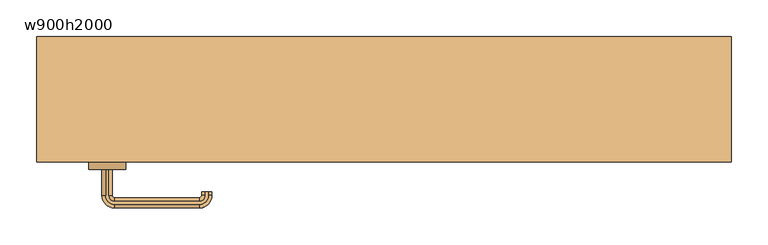
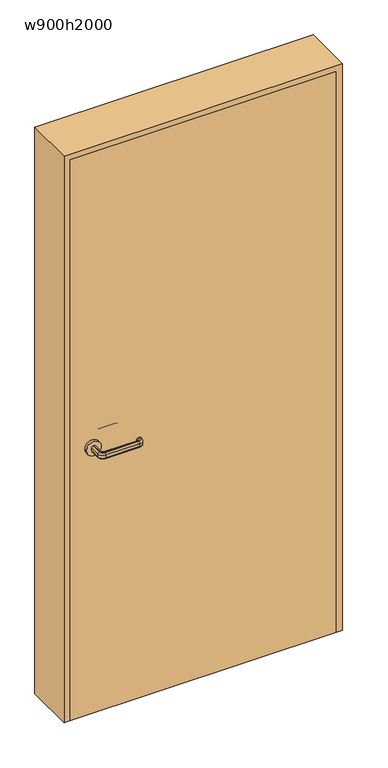
"""IFC4 building model written with IfcOpenShell, lengths in millimetres: door geometry, 片開き : w900h2000."""

import ifcopenshell
import ifcopenshell.guid

model = None  # the IFC model being written
_history = None  # IfcOwnerHistory: only IFC2X3 demands one
_inside = {}  # id of a spatial element -> (the spatial element, [elements in it])
_under = {}  # id of a project, library or spatial element -> (it, [spatial elements below it])
_declared = {}  # id of a project -> (the project, [libraries it declares])
_typed = {}  # id of a type object -> (the type object, [elements of that type])
_made_of = {}  # id of a material, layer set ... -> (it, [elements and type objects made of it])


def new_model(schema):
    """Start an empty IFC model of exactly this schema.

    Asked for "IFC4X3", IfcOpenShell would pick the latest addendum, in which some entities
    have other attributes; the version numbers below select the first issue.
    IFC2X3 requires an IfcOwnerHistory on every rooted entity: one is made here for all.
    """
    global model, _history
    if schema == "IFC4X3":
        model = ifcopenshell.file(schema_version=(4, 3, 0, 0))
    else:
        model = ifcopenshell.file(schema=schema)
    _inside.clear()
    _under.clear()
    _declared.clear()
    _typed.clear()
    _made_of.clear()
    _history = None
    if model.schema == "IFC2X3":
        org = make("IfcOrganization", Name="unknown")
        user = make(
            "IfcPersonAndOrganization",
            ThePerson=make("IfcPerson", FamilyName="unknown"),
            TheOrganization=org,
        )
        app = make(
            "IfcApplication",
            ApplicationDeveloper=org,
            Version="unknown",
            ApplicationFullName="unknown",
            ApplicationIdentifier="unknown",
        )
        _history = make(
            "IfcOwnerHistory",
            OwningUser=user,
            OwningApplication=app,
            ChangeAction="ADDED",
            CreationDate=0,
        )
    return model


def make(cls, **values):
    """One entity of the class cls with the attributes given. An attribute that is None is left unset."""
    return model.create_entity(
        cls, **{name: value for name, value in values.items() if value is not None}
    )


def rooted(cls, **values):
    """An entity with a GlobalId (a new one), such as an element, a storey or a relation."""
    return make(cls, GlobalId=ifcopenshell.guid.new(), OwnerHistory=_history, **values)


def si_unit(unit_type, name, prefix=None):
    """IfcSIUnit, for example si_unit("LENGTHUNIT", "METRE", prefix="MILLI")."""
    return make("IfcSIUnit", UnitType=unit_type, Prefix=prefix, Name=name)


def assignment(units):
    """IfcUnitAssignment: the units of a project."""
    return None if units is None else make("IfcUnitAssignment", Units=units)


def point(xyz):
    """IfcCartesianPoint."""
    return None if xyz is None else make("IfcCartesianPoint", Coordinates=xyz)


def direction(xyz):
    """IfcDirection."""
    return None if xyz is None else make("IfcDirection", DirectionRatios=xyz)


def frame(location, z_axis=None, x_axis=None):
    """IfcAxis2Placement3D, a coordinate frame: its origin and axes. An axis left out is left unset."""
    return make(
        "IfcAxis2Placement3D",
        Location=point(location),
        Axis=direction(z_axis),
        RefDirection=direction(x_axis),
    )


def frame_2d(location, x_axis=None):
    """IfcAxis2Placement2D, a coordinate frame in the plane: its origin and x axis."""
    return make(
        "IfcAxis2Placement2D", Location=point(location), RefDirection=direction(x_axis)
    )


def origin():
    """The frame at (0, 0, 0) with its axes left unset."""
    return frame((0.0, 0.0, 0.0))


def origin_with_axes():
    """The frame at (0, 0, 0) with the z axis (0, 0, 1) and the x axis (1, 0, 0) written out."""
    return frame((0.0, 0.0, 0.0), z_axis=(0.0, 0.0, 1.0), x_axis=(1.0, 0.0, 0.0))


def place(relative_to, where):
    """IfcLocalPlacement: puts the frame where relative to a parent placement (None: the world)."""
    return make(
        "IfcLocalPlacement", PlacementRelTo=relative_to, RelativePlacement=where
    )


def context(
    kind, dimensions, precision=None, world=None, true_north=None, identifier=None
):
    """IfcGeometricRepresentationContext, for example the 3D "Model" context."""
    return make(
        "IfcGeometricRepresentationContext",
        ContextIdentifier=identifier,
        ContextType=kind,
        CoordinateSpaceDimension=dimensions,
        Precision=precision,
        WorldCoordinateSystem=world,
        TrueNorth=true_north,
    )


def project(units=None, contexts=None):
    """IfcProject with its units and contexts."""
    return rooted(
        "IfcProject",
        Name="project",
        RepresentationContexts=contexts,
        UnitsInContext=assignment(units),
    )


def spatial(cls, under=None, at=None, **own):
    """A site, building, storey or space (cls), placed at a placement, below another one or the project."""
    s = rooted(cls, ObjectPlacement=at, **own)
    if under is not None:
        _under.setdefault(under.id(), (under, []))[1].append(s)
    return s


def polyline(points):
    """IfcPolyline through the points."""
    return make("IfcPolyline", Points=[point(p) for p in points])


def circle_curve(where, radius):
    """IfcCircle in the frame where."""
    return make("IfcCircle", Position=where, Radius=radius)


def ellipse_curve(where, semi_axis1, semi_axis2):
    """IfcEllipse in the frame where."""
    return make(
        "IfcEllipse", Position=where, SemiAxis1=semi_axis1, SemiAxis2=semi_axis2
    )


def trimmed(basis, trim1, trim2, sense, master):
    """IfcTrimmedCurve: the piece of a basis curve between two trims."""
    return make(
        "IfcTrimmedCurve",
        BasisCurve=basis,
        Trim1=trim1,
        Trim2=trim2,
        SenseAgreement=sense,
        MasterRepresentation=master,
    )


def segment(curve, same_sense, transition):
    """IfcCompositeCurveSegment."""
    return make(
        "IfcCompositeCurveSegment",
        Transition=transition,
        SameSense=same_sense,
        ParentCurve=curve,
    )


def composite_curve(segments, self_intersect=None):
    """IfcCompositeCurve: segments joined end to end."""
    return make("IfcCompositeCurve", Segments=segments, SelfIntersect=self_intersect)


def outline(outer, holes=None, kind="AREA"):
    """IfcArbitraryClosedProfileDef: a profile drawn as a closed curve; with holes, ...WithVoids."""
    if holes is None:
        return make("IfcArbitraryClosedProfileDef", ProfileType=kind, OuterCurve=outer)
    return make(
        "IfcArbitraryProfileDefWithVoids",
        ProfileType=kind,
        OuterCurve=outer,
        InnerCurves=holes,
    )


def extrude(swept, where, along, depth):
    """IfcExtrudedAreaSolid: the profile swept, set in the frame where, extruded along a direction by depth."""
    return make(
        "IfcExtrudedAreaSolid",
        SweptArea=swept,
        Position=where,
        ExtrudedDirection=direction(along),
        Depth=depth,
    )


def shape(context_of_items, identifier, shape_type, items):
    """IfcShapeRepresentation: the items that make up one representation, for example the "Body"."""
    return make(
        "IfcShapeRepresentation",
        ContextOfItems=context_of_items,
        RepresentationIdentifier=identifier,
        RepresentationType=shape_type,
        Items=items,
    )


def source(mapping_origin, context_of_items, identifier, shape_type, items):
    """IfcRepresentationMap: a shape defined once, which mapped items show again and again."""
    return make(
        "IfcRepresentationMap",
        MappingOrigin=mapping_origin,
        MappedRepresentation=shape(context_of_items, identifier, shape_type, items),
    )


def transform(
    local_origin,
    x_axis=None,
    y_axis=None,
    z_axis=None,
    scale=None,
    scale2=None,
    scale3=None,
    uniform=True,
):
    """IfcCartesianTransformationOperator3D, or its non-uniform kind. x_axis, y_axis, z_axis: its Axis1, 2, 3."""
    if uniform:
        return make(
            "IfcCartesianTransformationOperator3D",
            Axis1=direction(x_axis),
            Axis2=direction(y_axis),
            LocalOrigin=point(local_origin),
            Scale=scale,
            Axis3=direction(z_axis),
        )
    return make(
        "IfcCartesianTransformationOperator3DnonUniform",
        Axis1=direction(x_axis),
        Axis2=direction(y_axis),
        LocalOrigin=point(local_origin),
        Scale=scale,
        Axis3=direction(z_axis),
        Scale2=scale2,
        Scale3=scale3,
    )


def mapped(mapping_source, mapping_target):
    """IfcMappedItem: shows the shape of a source again, moved by a transform."""
    return make(
        "IfcMappedItem", MappingSource=mapping_source, MappingTarget=mapping_target
    )


def made_of(thing, what):
    """Note that an element or type object is made of a material, layer set ...; save() writes the relation."""
    if what is not None:
        _made_of.setdefault(what.id(), (what, []))[1].append(thing)
    return thing


def element(
    cls,
    number,
    at=None,
    inside=None,
    cuts=None,
    type_object=None,
    material=None,
    context=None,
    identifier="Body",
    shape_type=None,
    held_by="IfcProductDefinitionShape",
    body=None,
    shapes=None,
    **own,
):
    """One element of the class cls, such as IfcWall. Its Tag is "e" and its number.

    at: its placement. inside: the storey or other place that contains it. cuts: it is an
    opening in that element (IfcRelVoidsElement). A single representation is given by context,
    identifier, shape_type and body (its items); several are given by shapes. held_by: the class
    of the entity that holds the representations. save() writes the other relations.
    """
    e = rooted(cls, Tag="e%d" % number, ObjectPlacement=at, **own)
    if body is not None:
        shapes = [shape(context, identifier, shape_type, body)]
    if shapes is not None:
        e.Representation = make(held_by, Representations=shapes)
    if inside is not None:
        _inside.setdefault(inside.id(), (inside, []))[1].append(e)
    if cuts is not None:
        rooted(
            "IfcRelVoidsElement", RelatingBuildingElement=cuts, RelatedOpeningElement=e
        )
    if type_object is not None:
        _typed.setdefault(type_object.id(), (type_object, []))[1].append(e)
    return made_of(e, material)


def aggregate(whole, parts):
    """IfcRelAggregates: a whole, such as a stair, and the parts it consists of."""
    return rooted("IfcRelAggregates", RelatingObject=whole, RelatedObjects=parts)


def save(model, path):
    """Write the relations noted so far, then the file.

    IfcRelAggregates (storeys below a building ...), IfcRelContainedInSpatialStructure (elements
    in a storey), IfcRelDefinesByType, IfcRelAssociatesMaterial and IfcRelDeclares: one each for
    every whole, place, type object, material and project.
    """
    for whole, parts in _under.values():
        aggregate(whole, parts)
    for where, things in _inside.values():
        rooted(
            "IfcRelContainedInSpatialStructure",
            RelatedElements=things,
            RelatingStructure=where,
        )
    for kind, things in _typed.values():
        rooted("IfcRelDefinesByType", RelatedObjects=things, RelatingType=kind)
    for what, things in _made_of.values():
        rooted("IfcRelAssociatesMaterial", RelatedObjects=things, RelatingMaterial=what)
    for by, libraries in _declared.values():
        rooted("IfcRelDeclares", RelatingContext=by, RelatedDefinitions=libraries)
    model.write(path)


def plane_surface(at):
    """IfcPlane: the flat surface through the origin of the frame at, square to its z axis."""
    return make("IfcPlane", Position=at)


def cylinder_surface(at, radius):
    """IfcCylindricalSurface: all points at the distance radius from the z axis of the frame at."""
    return make("IfcCylindricalSurface", Position=at, Radius=radius)


def revolved_surface(curve, axis_point, axis_direction):
    """IfcSurfaceOfRevolution: the curve turned about the line through axis_point along axis_direction."""
    return make(
        "IfcSurfaceOfRevolution",
        SweptCurve=make("IfcArbitraryOpenProfileDef", ProfileType="CURVE", Curve=curve),
        AxisPosition=make("IfcAxis1Placement", Location=point(axis_point), Axis=direction(axis_direction)),
    )


def advanced_brep(points, edges, surfaces, faces):
    """IfcAdvancedBrep: a solid bounded by faces that lie on surfaces and meet in shared edges.

    An edge is (start, end): straight between two places in points (the first is 0);
    or (start, end, curve); or (start, end, curve, False) where it runs against its curve.
    A face is (place in surfaces, loops), or (place, loops, False) where it looks against
    its surface's normal. A loop lists edges by number (the first is 1), with a minus sign
    where the edge is run from its end to its start. The first loop is the outer one.
    """
    corners = [point(p) for p in points]
    vertices = [make("IfcVertexPoint", VertexGeometry=c) for c in corners]
    made = []
    for start, end, *more in edges:
        made.append(
            make(
                "IfcEdgeCurve",
                EdgeStart=vertices[start],
                EdgeEnd=vertices[end],
                EdgeGeometry=more[0] if more else make("IfcPolyline", Points=[corners[start], corners[end]]),
                SameSense=more[1] if len(more) > 1 else True,
            )
        )
    hull = []
    for where, loops, *sense in faces:
        bounds = []
        for j, loop in enumerate(loops):
            ring = [make("IfcOrientedEdge", EdgeElement=made[abs(k) - 1], Orientation=k > 0) for k in loop]
            bounds.append(
                make(
                    "IfcFaceOuterBound" if j == 0 else "IfcFaceBound",
                    Bound=make("IfcEdgeLoop", EdgeList=ring),
                    Orientation=True,
                )
            )
        hull.append(make("IfcAdvancedFace", Bounds=bounds, FaceSurface=surfaces[where], SameSense=sense[0] if sense else True))
    return make("IfcAdvancedBrep", Outer=make("IfcClosedShell", CfsFaces=hull))


def w900h2000_c063673d(model_context):
    return source(origin(), model_context, "Body", "SolidModel", [
        advanced_brep(
        [(-377.0, -95.0, 960.0), (-373.0, -95.0, 960.0), (-368.0, -95.0, 955.0), (-368.0, -95.0, 945.0477623), (-373.0, -95.0, 940.0477623), (-377.0, -95.0, 940.0477623), (-382.0, -95.0, 945.0477623), (-382.0, -95.0, 955.0), (-382.0, -130.0, 955.0), (-377.0, -130.0, 960.0), (-382.0, -130.0, 945.0477623), (-377.0, -130.0, 940.0477623), (-373.0, -130.0, 940.0477623), (-365.0, -138.0, 940.0477623), (-250.0, -138.0, 940.0477623), (-242.0, -130.0, 940.0477623), (-242.0, -125.0, 940.0477623), (-238.0, -125.0, 940.0477623), (-238.0, -130.0, 940.0477623), (-250.0, -142.0, 940.0477623), (-365.0, -142.0, 940.0477623), (-368.0, -130.0, 945.0477623), (-368.0, -130.0, 955.0), (-373.0, -130.0, 960.0), (-365.0, -142.0, 960.0), (-250.0, -142.0, 960.0), (-238.0, -130.0, 960.0), (-238.0, -125.0, 960.0), (-242.0, -125.0, 960.0), (-242.0, -130.0, 960.0), (-250.0, -138.0, 960.0), (-365.0, -138.0, 960.0), (-365.0, -147.0, 955.0), (-365.0, -147.0, 945.0477623), (-365.0, -133.0, 945.0477623), (-365.0, -133.0, 955.0), (-250.0, -147.0, 955.0), (-250.0, -147.0, 945.0477623), (-250.0, -133.0, 945.0477623), (-250.0, -133.0, 955.0), (-233.0, -130.0, 955.0), (-233.0, -130.0, 945.0477623), (-247.0, -130.0, 945.0477623), (-247.0, -130.0, 955.0), (-233.0, -125.0, 955.0), (-233.0, -125.0, 945.0477623), (-247.0, -125.0, 945.0477623), (-247.0, -125.0, 955.0)],
        [
            (0, 1),
            (1, 2, circle_curve(frame((-373.0, -95.0, 955.0), z_axis=(0.0, 1.0, 0.0), x_axis=(-1.0, 0.0, 0.0)), 5.0)),
            (2, 3),
            (3, 4, circle_curve(frame((-373.0, -95.0, 945.0477623), z_axis=(0.0, 1.0, 0.0), x_axis=(-1.0, 0.0, 0.0)), 5.0)),
            (4, 5),
            (5, 6, circle_curve(frame((-377.0, -95.0, 945.0477623), z_axis=(0.0, 1.0, 0.0), x_axis=(-1.0, 0.0, 0.0)), 5.0)),
            (6, 7),
            (7, 0, circle_curve(frame((-377.0, -95.0, 955.0), z_axis=(0.0, 1.0, 0.0), x_axis=(-1.0, 0.0, 0.0)), 5.0)),
            (7, 8),
            (8, 9, circle_curve(frame((-377.0, -130.0, 955.0), z_axis=(0.0, 1.0, 0.0), x_axis=(-1.0, 0.0, 0.0)), 5.0)),
            (9, 0),
            (6, 10),
            (10, 8),
            (5, 11),
            (11, 10, circle_curve(frame((-377.0, -130.0, 945.0477623), z_axis=(0.0, 1.0, 0.0), x_axis=(-1.0, 0.0, 0.0)), 5.0)),
            (4, 12),
            (12, 13, circle_curve(frame((-365.0, -130.0, 940.0477623), z_axis=(0.0, 0.0, 1.0), x_axis=(-1.0, 0.0, 0.0)), 8.0)),
            (13, 14),
            (14, 15, circle_curve(frame((-250.0, -130.0, 940.0477623), z_axis=(0.0, 0.0, 1.0), x_axis=(0.0, -1.0, 0.0)), 8.0)),
            (15, 16),
            (16, 17),
            (17, 18),
            (18, 19, circle_curve(frame((-250.0, -130.0, 940.0477623), z_axis=(0.0, 0.0, -1.0), x_axis=(0.0, -1.0, 0.0)), 12.0)),
            (19, 20),
            (20, 11, circle_curve(frame((-365.0, -130.0, 940.0477623), z_axis=(0.0, 0.0, -1.0), x_axis=(-1.0, 0.0, 0.0)), 12.0)),
            (3, 21),
            (21, 12, circle_curve(frame((-373.0, -130.0, 945.0477623), z_axis=(0.0, 1.0, 0.0), x_axis=(-1.0, 0.0, 0.0)), 5.0)),
            (2, 22),
            (22, 21),
            (1, 23),
            (23, 22, circle_curve(frame((-373.0, -130.0, 955.0), z_axis=(0.0, 1.0, 0.0), x_axis=(-1.0, 0.0, 0.0)), 5.0)),
            (9, 24, circle_curve(frame((-365.0, -130.0, 960.0), z_axis=(0.0, 0.0, 1.0), x_axis=(-1.0, 0.0, 0.0)), 12.0)),
            (24, 25),
            (25, 26, circle_curve(frame((-250.0, -130.0, 960.0), z_axis=(0.0, 0.0, 1.0), x_axis=(0.0, -1.0, 0.0)), 12.0)),
            (26, 27),
            (27, 28),
            (28, 29),
            (29, 30, circle_curve(frame((-250.0, -130.0, 960.0), z_axis=(0.0, 0.0, -1.0), x_axis=(0.0, -1.0, 0.0)), 8.0)),
            (30, 31),
            (31, 23, circle_curve(frame((-365.0, -130.0, 960.0), z_axis=(0.0, 0.0, -1.0), x_axis=(-1.0, 0.0, 0.0)), 8.0)),
            (32, 24, circle_curve(frame((-365.0, -142.0, 955.0), z_axis=(-1.0, 0.0, 0.0), x_axis=(0.0, -1.0, 0.0)), 5.0)),
            (8, 32, circle_curve(frame((-365.0, -130.0, 955.0), z_axis=(0.0, 0.0, 1.0), x_axis=(-1.0, 0.0, 0.0)), 17.0)),
            (33, 32),
            (10, 33, circle_curve(frame((-365.0, -130.0, 945.0477623), z_axis=(0.0, 0.0, 1.0), x_axis=(-1.0, 0.0, 0.0)), 17.0)),
            (20, 33, circle_curve(frame((-365.0, -142.0, 945.0477623), z_axis=(-1.0, 0.0, 0.0), x_axis=(0.0, -1.0, 0.0)), 5.0)),
            (34, 13, circle_curve(frame((-365.0, -138.0, 945.0477623), z_axis=(-1.0, 0.0, 0.0), x_axis=(0.0, -1.0, 0.0)), 5.0)),
            (21, 34, circle_curve(frame((-365.0, -130.0, 945.0477623), z_axis=(0.0, 0.0, 1.0), x_axis=(-1.0, 0.0, 0.0)), 3.0)),
            (35, 34),
            (22, 35, circle_curve(frame((-365.0, -130.0, 955.0), z_axis=(0.0, 0.0, 1.0), x_axis=(-1.0, 0.0, 0.0)), 3.0)),
            (31, 35, circle_curve(frame((-365.0, -138.0, 955.0), z_axis=(-1.0, 0.0, 0.0), x_axis=(0.0, -1.0, 0.0)), 5.0)),
            (32, 36),
            (36, 25, circle_curve(frame((-250.0, -142.0, 955.0), z_axis=(-1.0, 0.0, 0.0), x_axis=(0.0, -1.0, 0.0)), 5.0)),
            (33, 37),
            (37, 36),
            (19, 37, circle_curve(frame((-250.0, -142.0, 945.0477623), z_axis=(-1.0, 0.0, 0.0), x_axis=(0.0, -1.0, 0.0)), 5.0)),
            (34, 38),
            (38, 14, circle_curve(frame((-250.0, -138.0, 945.0477623), z_axis=(-1.0, 0.0, 0.0), x_axis=(0.0, -1.0, 0.0)), 5.0)),
            (35, 39),
            (39, 38),
            (30, 39, circle_curve(frame((-250.0, -138.0, 955.0), z_axis=(-1.0, 0.0, 0.0), x_axis=(0.0, -1.0, 0.0)), 5.0)),
            (40, 26, circle_curve(frame((-238.0, -130.0, 955.0), z_axis=(0.0, -1.0, 0.0), x_axis=(1.0, 0.0, 0.0)), 5.0)),
            (36, 40, circle_curve(frame((-250.0, -130.0, 955.0), z_axis=(0.0, 0.0, 1.0), x_axis=(0.0, -1.0, 0.0)), 17.0)),
            (41, 40),
            (37, 41, circle_curve(frame((-250.0, -130.0, 945.0477623), z_axis=(0.0, 0.0, 1.0), x_axis=(0.0, -1.0, 0.0)), 17.0)),
            (18, 41, circle_curve(frame((-238.0, -130.0, 945.0477623), z_axis=(0.0, -1.0, 0.0), x_axis=(1.0, 0.0, 0.0)), 5.0)),
            (42, 15, circle_curve(frame((-242.0, -130.0, 945.0477623), z_axis=(0.0, -1.0, 0.0), x_axis=(1.0, 0.0, 0.0)), 5.0)),
            (38, 42, circle_curve(frame((-250.0, -130.0, 945.0477623), z_axis=(0.0, 0.0, 1.0), x_axis=(0.0, -1.0, 0.0)), 3.0)),
            (43, 42),
            (39, 43, circle_curve(frame((-250.0, -130.0, 955.0), z_axis=(0.0, 0.0, 1.0), x_axis=(0.0, -1.0, 0.0)), 3.0)),
            (29, 43, circle_curve(frame((-242.0, -130.0, 955.0), z_axis=(0.0, -1.0, 0.0), x_axis=(1.0, 0.0, 0.0)), 5.0)),
            (27, 44, circle_curve(frame((-238.0, -125.0, 955.0), z_axis=(0.0, 1.0, 0.0), x_axis=(1.0, 0.0, 0.0)), 5.0)),
            (44, 45),
            (45, 17, circle_curve(frame((-238.0, -125.0, 945.0477623), z_axis=(0.0, 1.0, 0.0), x_axis=(1.0, 0.0, 0.0)), 5.0)),
            (16, 46, circle_curve(frame((-242.0, -125.0, 945.0477623), z_axis=(0.0, 1.0, 0.0), x_axis=(1.0, 0.0, 0.0)), 5.0)),
            (46, 47),
            (47, 28, circle_curve(frame((-242.0, -125.0, 955.0), z_axis=(0.0, 1.0, 0.0), x_axis=(1.0, 0.0, 0.0)), 5.0)),
            (40, 44),
            (41, 45),
            (42, 46),
            (43, 47),
        ],
        [
            plane_surface(frame((-385.198039, -95.0, 950.0), z_axis=(0.0, 1.0, 0.0), x_axis=(0.0, 0.0, 1.0))),
            cylinder_surface(frame((-377.0, -95.0, 955.0), z_axis=(0.0, 1.0, 0.0), x_axis=(-1.0, 0.0, 0.0)), 5.0),
            plane_surface(frame((-382.0, -95.0, 955.0), z_axis=(-1.0, 0.0, 0.0), x_axis=(0.0, -1.0, 0.0))),
            cylinder_surface(frame((-377.0, -95.0, 945.0477623), z_axis=(0.0, 1.0, 0.0), x_axis=(-1.0, 0.0, 0.0)), 5.0),
            plane_surface(frame((-377.0, -95.0, 940.0477623), z_axis=(0.0, 0.0, -1.0), x_axis=(0.0, -1.0, 0.0))),
            cylinder_surface(frame((-373.0, -95.0, 945.0477623), z_axis=(0.0, 1.0, 0.0), x_axis=(-1.0, 0.0, 0.0)), 5.0),
            plane_surface(frame((-368.0, -95.0, 945.0477623), z_axis=(1.0, 0.0, 0.0), x_axis=(0.0, -1.0, 0.0))),
            cylinder_surface(frame((-373.0, -95.0, 955.0), z_axis=(0.0, 1.0, 0.0), x_axis=(-1.0, 0.0, 0.0)), 5.0),
            plane_surface(frame((-373.0, -95.0, 960.0), z_axis=(0.0, 0.0, 1.0), x_axis=(0.0, -1.0, 0.0))),
            revolved_surface(trimmed(ellipse_curve(frame((-377.0, -130.0, 955.0), z_axis=(0.0, -1.0, 0.0), x_axis=(-1.0, 0.0, 0.0)), 5.0, 5.0), [point((-377.0, -130.0, 960.0))], [point((-382.0, -130.0, 955.0))], True, "CARTESIAN"), (-365.0, -130.0, 950.0), (0.0, 0.0, -1.0)),
            cylinder_surface(frame((-365.0, -130.0, 950.0), z_axis=(0.0, 0.0, -1.0), x_axis=(-1.0, 0.0, 0.0)), 17.0),
            revolved_surface(trimmed(ellipse_curve(frame((-377.0, -130.0, 945.0477623), z_axis=(0.0, -1.0, 0.0), x_axis=(-1.0, 0.0, 0.0)), 5.0, 5.0), [point((-382.0, -130.0, 945.0477623))], [point((-377.0, -130.0, 940.0477623))], True, "CARTESIAN"), (-365.0, -130.0, 950.0), (0.0, 0.0, -1.0)),
            revolved_surface(trimmed(ellipse_curve(frame((-373.0, -130.0, 945.0477623), z_axis=(0.0, -1.0, 0.0), x_axis=(-1.0, 0.0, 0.0)), 5.0, 5.0), [point((-373.0, -130.0, 940.0477623))], [point((-368.0, -130.0, 945.0477623))], True, "CARTESIAN"), (-365.0, -130.0, 950.0), (0.0, 0.0, -1.0)),
            revolved_surface(polyline([(-368.0, -130.0, 945.0477623), (-368.0, -130.0, 955.0)]), (-365.0, -130.0, 950.0), (0.0, 0.0, -1.0)),
            revolved_surface(trimmed(ellipse_curve(frame((-373.0, -130.0, 955.0), z_axis=(0.0, -1.0, 0.0), x_axis=(-1.0, 0.0, 0.0)), 5.0, 5.0), [point((-368.0, -130.0, 955.0))], [point((-373.0, -130.0, 960.0))], True, "CARTESIAN"), (-365.0, -130.0, 950.0), (0.0, 0.0, -1.0)),
            cylinder_surface(frame((-365.0, -142.0, 955.0), z_axis=(-1.0, 0.0, 0.0), x_axis=(0.0, -1.0, 0.0)), 5.0),
            plane_surface(frame((-365.0, -147.0, 955.0), z_axis=(0.0, -1.0, 0.0), x_axis=(1.0, 0.0, 0.0))),
            cylinder_surface(frame((-365.0, -142.0, 945.0477623), z_axis=(-1.0, 0.0, 0.0), x_axis=(0.0, -1.0, 0.0)), 5.0),
            cylinder_surface(frame((-365.0, -138.0, 945.0477623), z_axis=(-1.0, 0.0, 0.0), x_axis=(0.0, -1.0, 0.0)), 5.0),
            plane_surface(frame((-365.0, -133.0, 945.0477623), z_axis=(0.0, 1.0, 0.0), x_axis=(1.0, 0.0, 0.0))),
            cylinder_surface(frame((-365.0, -138.0, 955.0), z_axis=(-1.0, 0.0, 0.0), x_axis=(0.0, -1.0, 0.0)), 5.0),
            revolved_surface(trimmed(ellipse_curve(frame((-250.0, -142.0, 955.0), z_axis=(1.0, 0.0, 0.0), x_axis=(0.0, -1.0, 0.0)), 5.0, 5.0), [point((-250.0, -142.0, 960.0))], [point((-250.0, -147.0, 955.0))], True, "CARTESIAN"), (-250.0, -130.0, 950.0), (0.0, 0.0, -1.0)),
            cylinder_surface(frame((-250.0, -130.0, 950.0), z_axis=(0.0, 0.0, -1.0), x_axis=(0.0, -1.0, 0.0)), 17.0),
            revolved_surface(trimmed(ellipse_curve(frame((-250.0, -142.0, 945.0477623), z_axis=(1.0, 0.0, 0.0), x_axis=(0.0, -1.0, 0.0)), 5.0, 5.0), [point((-250.0, -147.0, 945.0477623))], [point((-250.0, -142.0, 940.0477623))], True, "CARTESIAN"), (-250.0, -130.0, 950.0), (0.0, 0.0, -1.0)),
            revolved_surface(trimmed(ellipse_curve(frame((-250.0, -138.0, 945.0477623), z_axis=(1.0, 0.0, 0.0), x_axis=(0.0, -1.0, 0.0)), 5.0, 5.0), [point((-250.0, -138.0, 940.0477623))], [point((-250.0, -133.0, 945.0477623))], True, "CARTESIAN"), (-250.0, -130.0, 950.0), (0.0, 0.0, -1.0)),
            revolved_surface(polyline([(-250.0, -133.0, 945.0477623), (-250.0, -133.0, 955.0)]), (-250.0, -130.0, 950.0), (0.0, 0.0, -1.0)),
            revolved_surface(trimmed(ellipse_curve(frame((-250.0, -138.0, 955.0), z_axis=(1.0, 0.0, 0.0), x_axis=(0.0, -1.0, 0.0)), 5.0, 5.0), [point((-250.0, -133.0, 955.0))], [point((-250.0, -138.0, 960.0))], True, "CARTESIAN"), (-250.0, -130.0, 950.0), (0.0, 0.0, -1.0)),
            plane_surface(frame((-250.198039, -125.0, 950.0), z_axis=(0.0, 1.0, 0.0), x_axis=(0.0, 0.0, -1.0))),
            cylinder_surface(frame((-238.0, -130.0, 955.0), z_axis=(0.0, -1.0, 0.0), x_axis=(1.0, 0.0, 0.0)), 5.0),
            plane_surface(frame((-233.0, -130.0, 955.0), z_axis=(1.0, 0.0, 0.0), x_axis=(0.0, 1.0, 0.0))),
            cylinder_surface(frame((-238.0, -130.0, 945.0477623), z_axis=(0.0, -1.0, 0.0), x_axis=(1.0, 0.0, 0.0)), 5.0),
            cylinder_surface(frame((-242.0, -130.0, 945.0477623), z_axis=(0.0, -1.0, 0.0), x_axis=(1.0, 0.0, 0.0)), 5.0),
            plane_surface(frame((-247.0, -130.0, 945.0477623), z_axis=(-1.0, 0.0, 0.0), x_axis=(0.0, 1.0, 0.0))),
            cylinder_surface(frame((-242.0, -130.0, 955.0), z_axis=(0.0, -1.0, 0.0), x_axis=(1.0, 0.0, 0.0)), 5.0),
        ],
        [
            (0, [[1, 2, 3, 4, 5, 6, 7, 8]]),
            (1, [[9, 10, 11, -8]]),
            (2, [[12, 13, -9, -7]]),
            (3, [[14, 15, -12, -6]]),
            (4, [[16, 17, 18, 19, 20, 21, 22, 23, 24, 25, -14, -5]]),
            (5, [[26, 27, -16, -4]]),
            (6, [[28, 29, -26, -3]]),
            (7, [[30, 31, -28, -2]]),
            (8, [[-11, 32, 33, 34, 35, 36, 37, 38, 39, 40, -30, -1]]),
            (9, [[41, -32, -10, 42]]),
            (10, [[43, -42, -13, 44]]),
            (11, [[45, -44, -15, -25]]),
            (12, [[46, -17, -27, 47]]),
            (13, [[48, -47, -29, 49]]),
            (14, [[50, -49, -31, -40]]),
            (15, [[51, 52, -33, -41]]),
            (16, [[53, 54, -51, -43]]),
            (17, [[-24, 55, -53, -45]]),
            (18, [[56, 57, -18, -46]]),
            (19, [[58, 59, -56, -48]]),
            (20, [[-39, 60, -58, -50]]),
            (21, [[61, -34, -52, 62]]),
            (22, [[63, -62, -54, 64]]),
            (23, [[65, -64, -55, -23]]),
            (24, [[66, -19, -57, 67]]),
            (25, [[68, -67, -59, 69]]),
            (26, [[70, -69, -60, -38]]),
            (27, [[71, 72, 73, -21, 74, 75, 76, -36]]),
            (28, [[77, -71, -35, -61]]),
            (29, [[78, -72, -77, -63]]),
            (30, [[-22, -73, -78, -65]]),
            (31, [[79, -74, -20, -66]]),
            (32, [[80, -75, -79, -68]]),
            (33, [[-37, -76, -80, -70]]),
        ],
    ),
        advanced_brep(
        [(-373.0, -45.0, 940.0), (-368.0, -45.0, 945.0), (-368.0, -45.0, 955.0), (-373.0, -45.0, 960.0), (-377.0, -45.0, 960.0), (-382.0, -45.0, 955.0), (-382.0, -45.0, 945.0), (-377.0, -45.0, 940.0), (-377.0, -10.0, 940.0), (-365.0, 2.0, 940.0), (-250.0, 2.0, 940.0), (-238.0, -10.0, 940.0), (-238.0, -15.0, 940.0), (-242.0, -15.0, 940.0), (-242.0, -10.0, 940.0), (-250.0, -2.0, 940.0), (-365.0, -2.0, 940.0), (-373.0, -10.0, 940.0), (-382.0, -10.0, 945.0), (-382.0, -10.0, 955.0), (-377.0, -10.0, 960.0), (-373.0, -10.0, 960.0), (-365.0, -2.0, 960.0), (-250.0, -2.0, 960.0), (-242.0, -10.0, 960.0), (-242.0, -15.0, 960.0), (-238.0, -15.0, 960.0), (-238.0, -10.0, 960.0), (-250.0, 2.0, 960.0), (-365.0, 2.0, 960.0), (-368.0, -10.0, 955.0), (-368.0, -10.0, 945.0), (-365.0, 7.0, 945.0), (-365.0, 7.0, 955.0), (-365.0, -7.0, 955.0), (-365.0, -7.0, 945.0), (-250.0, 7.0, 945.0), (-250.0, 7.0, 955.0), (-250.0, -7.0, 955.0), (-250.0, -7.0, 945.0), (-233.0, -10.0, 945.0), (-233.0, -10.0, 955.0), (-247.0, -10.0, 955.0), (-247.0, -10.0, 945.0), (-233.0, -15.0, 945.0), (-233.0, -15.0, 955.0), (-247.0, -15.0, 955.0), (-247.0, -15.0, 945.0)],
        [
            (0, 1, circle_curve(frame((-373.0, -45.0, 945.0), z_axis=(0.0, -1.0, 0.0), x_axis=(1.0, 0.0, 0.0)), 5.0)),
            (1, 2),
            (2, 3, circle_curve(frame((-373.0, -45.0, 955.0), z_axis=(0.0, -1.0, 0.0), x_axis=(1.0, 0.0, 0.0)), 5.0)),
            (3, 4),
            (4, 5, circle_curve(frame((-377.0, -45.0, 955.0), z_axis=(0.0, -1.0, 0.0), x_axis=(1.0, 0.0, 0.0)), 5.0)),
            (5, 6),
            (6, 7, circle_curve(frame((-377.0, -45.0, 945.0), z_axis=(0.0, -1.0, 0.0), x_axis=(1.0, 0.0, 0.0)), 5.0)),
            (7, 0),
            (7, 8),
            (8, 9, circle_curve(frame((-365.0, -10.0, 940.0), z_axis=(0.0, 0.0, -1.0), x_axis=(-1.0, 0.0, 0.0)), 12.0)),
            (9, 10),
            (10, 11, circle_curve(frame((-250.0, -10.0, 940.0), z_axis=(0.0, 0.0, -1.0), x_axis=(0.0, 1.0, 0.0)), 12.0)),
            (11, 12),
            (12, 13),
            (13, 14),
            (14, 15, circle_curve(frame((-250.0, -10.0, 940.0), z_axis=(0.0, 0.0, 1.0), x_axis=(0.0, 1.0, 0.0)), 8.0)),
            (15, 16),
            (16, 17, circle_curve(frame((-365.0, -10.0, 940.0), z_axis=(0.0, 0.0, 1.0), x_axis=(-1.0, 0.0, 0.0)), 8.0)),
            (17, 0),
            (6, 18),
            (18, 8, circle_curve(frame((-377.0, -10.0, 945.0), z_axis=(0.0, -1.0, 0.0), x_axis=(1.0, 0.0, 0.0)), 5.0)),
            (5, 19),
            (19, 18),
            (4, 20),
            (20, 19, circle_curve(frame((-377.0, -10.0, 955.0), z_axis=(0.0, -1.0, 0.0), x_axis=(1.0, 0.0, 0.0)), 5.0)),
            (3, 21),
            (21, 22, circle_curve(frame((-365.0, -10.0, 960.0), z_axis=(0.0, 0.0, -1.0), x_axis=(-1.0, 0.0, 0.0)), 8.0)),
            (22, 23),
            (23, 24, circle_curve(frame((-250.0, -10.0, 960.0), z_axis=(0.0, 0.0, -1.0), x_axis=(0.0, 1.0, 0.0)), 8.0)),
            (24, 25),
            (25, 26),
            (26, 27),
            (27, 28, circle_curve(frame((-250.0, -10.0, 960.0), z_axis=(0.0, 0.0, 1.0), x_axis=(0.0, 1.0, 0.0)), 12.0)),
            (28, 29),
            (29, 20, circle_curve(frame((-365.0, -10.0, 960.0), z_axis=(0.0, 0.0, 1.0), x_axis=(-1.0, 0.0, 0.0)), 12.0)),
            (2, 30),
            (30, 21, circle_curve(frame((-373.0, -10.0, 955.0), z_axis=(0.0, -1.0, 0.0), x_axis=(1.0, 0.0, 0.0)), 5.0)),
            (1, 31),
            (31, 30),
            (17, 31, circle_curve(frame((-373.0, -10.0, 945.0), z_axis=(0.0, -1.0, 0.0), x_axis=(1.0, 0.0, 0.0)), 5.0)),
            (32, 9, circle_curve(frame((-365.0, 2.0, 945.0), z_axis=(-1.0, 0.0, 0.0), x_axis=(0.0, -1.0, 0.0)), 5.0)),
            (18, 32, circle_curve(frame((-365.0, -10.0, 945.0), z_axis=(0.0, 0.0, -1.0), x_axis=(-1.0, 0.0, 0.0)), 17.0)),
            (33, 32),
            (19, 33, circle_curve(frame((-365.0, -10.0, 955.0), z_axis=(0.0, 0.0, -1.0), x_axis=(-1.0, 0.0, 0.0)), 17.0)),
            (29, 33, circle_curve(frame((-365.0, 2.0, 955.0), z_axis=(-1.0, 0.0, 0.0), x_axis=(0.0, -1.0, 0.0)), 5.0)),
            (34, 22, circle_curve(frame((-365.0, -2.0, 955.0), z_axis=(-1.0, 0.0, 0.0), x_axis=(0.0, -1.0, 0.0)), 5.0)),
            (30, 34, circle_curve(frame((-365.0, -10.0, 955.0), z_axis=(0.0, 0.0, -1.0), x_axis=(-1.0, 0.0, 0.0)), 3.0)),
            (35, 34),
            (31, 35, circle_curve(frame((-365.0, -10.0, 945.0), z_axis=(0.0, 0.0, -1.0), x_axis=(-1.0, 0.0, 0.0)), 3.0)),
            (16, 35, circle_curve(frame((-365.0, -2.0, 945.0), z_axis=(-1.0, 0.0, 0.0), x_axis=(0.0, -1.0, 0.0)), 5.0)),
            (32, 36),
            (36, 10, circle_curve(frame((-250.0, 2.0, 945.0), z_axis=(-1.0, 0.0, 0.0), x_axis=(0.0, -1.0, 0.0)), 5.0)),
            (33, 37),
            (37, 36),
            (28, 37, circle_curve(frame((-250.0, 2.0, 955.0), z_axis=(-1.0, 0.0, 0.0), x_axis=(0.0, -1.0, 0.0)), 5.0)),
            (34, 38),
            (38, 23, circle_curve(frame((-250.0, -2.0, 955.0), z_axis=(-1.0, 0.0, 0.0), x_axis=(0.0, -1.0, 0.0)), 5.0)),
            (35, 39),
            (39, 38),
            (15, 39, circle_curve(frame((-250.0, -2.0, 945.0), z_axis=(-1.0, 0.0, 0.0), x_axis=(0.0, -1.0, 0.0)), 5.0)),
            (40, 11, circle_curve(frame((-238.0, -10.0, 945.0), z_axis=(0.0, 1.0, 0.0), x_axis=(-1.0, 0.0, 0.0)), 5.0)),
            (36, 40, circle_curve(frame((-250.0, -10.0, 945.0), z_axis=(0.0, 0.0, -1.0), x_axis=(0.0, 1.0, 0.0)), 17.0)),
            (41, 40),
            (37, 41, circle_curve(frame((-250.0, -10.0, 955.0), z_axis=(0.0, 0.0, -1.0), x_axis=(0.0, 1.0, 0.0)), 17.0)),
            (27, 41, circle_curve(frame((-238.0, -10.0, 955.0), z_axis=(0.0, 1.0, 0.0), x_axis=(-1.0, 0.0, 0.0)), 5.0)),
            (42, 24, circle_curve(frame((-242.0, -10.0, 955.0), z_axis=(0.0, 1.0, 0.0), x_axis=(-1.0, 0.0, 0.0)), 5.0)),
            (38, 42, circle_curve(frame((-250.0, -10.0, 955.0), z_axis=(0.0, 0.0, -1.0), x_axis=(0.0, 1.0, 0.0)), 3.0)),
            (43, 42),
            (39, 43, circle_curve(frame((-250.0, -10.0, 945.0), z_axis=(0.0, 0.0, -1.0), x_axis=(0.0, 1.0, 0.0)), 3.0)),
            (14, 43, circle_curve(frame((-242.0, -10.0, 945.0), z_axis=(0.0, 1.0, 0.0), x_axis=(-1.0, 0.0, 0.0)), 5.0)),
            (12, 44, circle_curve(frame((-238.0, -15.0, 945.0), z_axis=(0.0, -1.0, 0.0), x_axis=(-1.0, 0.0, 0.0)), 5.0)),
            (44, 45),
            (45, 26, circle_curve(frame((-238.0, -15.0, 955.0), z_axis=(0.0, -1.0, 0.0), x_axis=(-1.0, 0.0, 0.0)), 5.0)),
            (25, 46, circle_curve(frame((-242.0, -15.0, 955.0), z_axis=(0.0, -1.0, 0.0), x_axis=(-1.0, 0.0, 0.0)), 5.0)),
            (46, 47),
            (47, 13, circle_curve(frame((-242.0, -15.0, 945.0), z_axis=(0.0, -1.0, 0.0), x_axis=(-1.0, 0.0, 0.0)), 5.0)),
            (40, 44),
            (41, 45),
            (42, 46),
            (43, 47),
        ],
        [
            plane_surface(frame((-385.198039, -45.0, 950.0), z_axis=(0.0, -1.0, 0.0), x_axis=(0.0, 0.0, -1.0))),
            plane_surface(frame((-373.0, -45.0, 940.0), z_axis=(0.0, 0.0, -1.0), x_axis=(0.0, 1.0, 0.0))),
            cylinder_surface(frame((-377.0, -45.0, 945.0), z_axis=(0.0, -1.0, 0.0), x_axis=(1.0, 0.0, 0.0)), 5.0),
            plane_surface(frame((-382.0, -45.0, 945.0), z_axis=(-1.0, 0.0, 0.0), x_axis=(0.0, 1.0, 0.0))),
            cylinder_surface(frame((-377.0, -45.0, 955.0), z_axis=(0.0, -1.0, 0.0), x_axis=(1.0, 0.0, 0.0)), 5.0),
            plane_surface(frame((-377.0, -45.0, 960.0), z_axis=(0.0, 0.0, 1.0), x_axis=(0.0, 1.0, 0.0))),
            cylinder_surface(frame((-373.0, -45.0, 955.0), z_axis=(0.0, -1.0, 0.0), x_axis=(1.0, 0.0, 0.0)), 5.0),
            plane_surface(frame((-368.0, -45.0, 955.0), z_axis=(1.0, 0.0, 0.0), x_axis=(0.0, 1.0, 0.0))),
            cylinder_surface(frame((-373.0, -45.0, 945.0), z_axis=(0.0, -1.0, 0.0), x_axis=(1.0, 0.0, 0.0)), 5.0),
            revolved_surface(trimmed(ellipse_curve(frame((-377.0, -10.0, 945.0), z_axis=(0.0, 1.0, 0.0), x_axis=(1.0, 0.0, 0.0)), 5.0, 5.0), [point((-377.0, -10.0, 940.0))], [point((-382.0, -10.0, 945.0))], True, "CARTESIAN"), (-365.0, -10.0, 950.0), (0.0, 0.0, 1.0)),
            cylinder_surface(frame((-365.0, -10.0, 950.0), z_axis=(0.0, 0.0, 1.0), x_axis=(-1.0, 0.0, 0.0)), 17.0),
            revolved_surface(trimmed(ellipse_curve(frame((-377.0, -10.0, 955.0), z_axis=(0.0, 1.0, 0.0), x_axis=(1.0, 0.0, 0.0)), 5.0, 5.0), [point((-382.0, -10.0, 955.0))], [point((-377.0, -10.0, 960.0))], True, "CARTESIAN"), (-365.0, -10.0, 950.0), (0.0, 0.0, 1.0)),
            revolved_surface(trimmed(ellipse_curve(frame((-373.0, -10.0, 955.0), z_axis=(0.0, 1.0, 0.0), x_axis=(1.0, 0.0, 0.0)), 5.0, 5.0), [point((-373.0, -10.0, 960.0))], [point((-368.0, -10.0, 955.0))], True, "CARTESIAN"), (-365.0, -10.0, 950.0), (0.0, 0.0, 1.0)),
            revolved_surface(polyline([(-368.0, -10.0, 955.0), (-368.0, -10.0, 945.0)]), (-365.0, -10.0, 950.0), (0.0, 0.0, 1.0)),
            revolved_surface(trimmed(ellipse_curve(frame((-373.0, -10.0, 945.0), z_axis=(0.0, 1.0, 0.0), x_axis=(1.0, 0.0, 0.0)), 5.0, 5.0), [point((-368.0, -10.0, 945.0))], [point((-373.0, -10.0, 940.0))], True, "CARTESIAN"), (-365.0, -10.0, 950.0), (0.0, 0.0, 1.0)),
            cylinder_surface(frame((-365.0, 2.0, 945.0), z_axis=(-1.0, 0.0, 0.0), x_axis=(0.0, -1.0, 0.0)), 5.0),
            plane_surface(frame((-365.0, 7.0, 945.0), z_axis=(0.0, 1.0, 0.0), x_axis=(1.0, 0.0, 0.0))),
            cylinder_surface(frame((-365.0, 2.0, 955.0), z_axis=(-1.0, 0.0, 0.0), x_axis=(0.0, -1.0, 0.0)), 5.0),
            cylinder_surface(frame((-365.0, -2.0, 955.0), z_axis=(-1.0, 0.0, 0.0), x_axis=(0.0, -1.0, 0.0)), 5.0),
            plane_surface(frame((-365.0, -7.0, 955.0), z_axis=(0.0, -1.0, 0.0), x_axis=(1.0, 0.0, 0.0))),
            cylinder_surface(frame((-365.0, -2.0, 945.0), z_axis=(-1.0, 0.0, 0.0), x_axis=(0.0, -1.0, 0.0)), 5.0),
            revolved_surface(trimmed(ellipse_curve(frame((-250.0, 2.0, 945.0), z_axis=(1.0, 0.0, 0.0), x_axis=(0.0, -1.0, 0.0)), 5.0, 5.0), [point((-250.0, 2.0, 940.0))], [point((-250.0, 7.0, 945.0))], True, "CARTESIAN"), (-250.0, -10.0, 950.0), (0.0, 0.0, 1.0)),
            cylinder_surface(frame((-250.0, -10.0, 950.0), z_axis=(0.0, 0.0, 1.0), x_axis=(0.0, 1.0, 0.0)), 17.0),
            revolved_surface(trimmed(ellipse_curve(frame((-250.0, 2.0, 955.0), z_axis=(1.0, 0.0, 0.0), x_axis=(0.0, -1.0, 0.0)), 5.0, 5.0), [point((-250.0, 7.0, 955.0))], [point((-250.0, 2.0, 960.0))], True, "CARTESIAN"), (-250.0, -10.0, 950.0), (0.0, 0.0, 1.0)),
            revolved_surface(trimmed(ellipse_curve(frame((-250.0, -2.0, 955.0), z_axis=(1.0, 0.0, 0.0), x_axis=(0.0, -1.0, 0.0)), 5.0, 5.0), [point((-250.0, -2.0, 960.0))], [point((-250.0, -7.0, 955.0))], True, "CARTESIAN"), (-250.0, -10.0, 950.0), (0.0, 0.0, 1.0)),
            revolved_surface(polyline([(-250.0, -7.0, 955.0), (-250.0, -7.0, 945.0)]), (-250.0, -10.0, 950.0), (0.0, 0.0, 1.0)),
            revolved_surface(trimmed(ellipse_curve(frame((-250.0, -2.0, 945.0), z_axis=(1.0, 0.0, 0.0), x_axis=(0.0, -1.0, 0.0)), 5.0, 5.0), [point((-250.0, -7.0, 945.0))], [point((-250.0, -2.0, 940.0))], True, "CARTESIAN"), (-250.0, -10.0, 950.0), (0.0, 0.0, 1.0)),
            plane_surface(frame((-250.198039, -15.0, 950.0), z_axis=(0.0, -1.0, 0.0), x_axis=(0.0, 0.0, 1.0))),
            cylinder_surface(frame((-238.0, -10.0, 945.0), z_axis=(0.0, 1.0, 0.0), x_axis=(-1.0, 0.0, 0.0)), 5.0),
            plane_surface(frame((-233.0, -10.0, 945.0), z_axis=(1.0, 0.0, 0.0), x_axis=(0.0, -1.0, 0.0))),
            cylinder_surface(frame((-238.0, -10.0, 955.0), z_axis=(0.0, 1.0, 0.0), x_axis=(-1.0, 0.0, 0.0)), 5.0),
            cylinder_surface(frame((-242.0, -10.0, 955.0), z_axis=(0.0, 1.0, 0.0), x_axis=(-1.0, 0.0, 0.0)), 5.0),
            plane_surface(frame((-247.0, -10.0, 955.0), z_axis=(-1.0, 0.0, 0.0), x_axis=(0.0, -1.0, 0.0))),
            cylinder_surface(frame((-242.0, -10.0, 945.0), z_axis=(0.0, 1.0, 0.0), x_axis=(-1.0, 0.0, 0.0)), 5.0),
        ],
        [
            (0, [[1, 2, 3, 4, 5, 6, 7, 8]]),
            (1, [[9, 10, 11, 12, 13, 14, 15, 16, 17, 18, 19, -8]]),
            (2, [[20, 21, -9, -7]]),
            (3, [[22, 23, -20, -6]]),
            (4, [[24, 25, -22, -5]]),
            (5, [[26, 27, 28, 29, 30, 31, 32, 33, 34, 35, -24, -4]]),
            (6, [[36, 37, -26, -3]]),
            (7, [[38, 39, -36, -2]]),
            (8, [[-19, 40, -38, -1]]),
            (9, [[41, -10, -21, 42]]),
            (10, [[43, -42, -23, 44]]),
            (11, [[45, -44, -25, -35]]),
            (12, [[46, -27, -37, 47]]),
            (13, [[48, -47, -39, 49]]),
            (14, [[50, -49, -40, -18]]),
            (15, [[51, 52, -11, -41]]),
            (16, [[53, 54, -51, -43]]),
            (17, [[-34, 55, -53, -45]]),
            (18, [[56, 57, -28, -46]]),
            (19, [[58, 59, -56, -48]]),
            (20, [[-17, 60, -58, -50]]),
            (21, [[61, -12, -52, 62]]),
            (22, [[63, -62, -54, 64]]),
            (23, [[65, -64, -55, -33]]),
            (24, [[66, -29, -57, 67]]),
            (25, [[68, -67, -59, 69]]),
            (26, [[70, -69, -60, -16]]),
            (27, [[-14, 71, 72, 73, -31, 74, 75, 76]]),
            (28, [[77, -71, -13, -61]]),
            (29, [[78, -72, -77, -63]]),
            (30, [[-32, -73, -78, -65]]),
            (31, [[79, -74, -30, -66]]),
            (32, [[80, -75, -79, -68]]),
            (33, [[-15, -76, -80, -70]]),
        ],
    ),
        extrude(outline(composite_curve([segment(trimmed(circle_curve(frame_2d((950.0, -375.0)), 25.0), [point((950.0, -400.0))], [point((950.0, -350.0))], False, "CARTESIAN"), True, "CONTINUOUS"), segment(trimmed(circle_curve(frame_2d((950.0, -375.0)), 25.0), [point((950.0, -350.0))], [point((950.0, -400.0))], False, "CARTESIAN"), True, "CONTINUOUS")], self_intersect=False)), frame((0.0, -95.0, 0.0), z_axis=(0.0, 1.0, 0.0), x_axis=(0.0, 0.0, 1.0)), (0.0, 0.0, 1.0), 10.0),
        extrude(outline(composite_curve([segment(trimmed(circle_curve(frame_2d((950.0, -375.0)), 25.0), [point((950.0, -400.0))], [point((950.0, -350.0))], False, "CARTESIAN"), True, "CONTINUOUS"), segment(trimmed(circle_curve(frame_2d((950.0, -375.0)), 25.0), [point((950.0, -350.0))], [point((950.0, -400.0))], False, "CARTESIAN"), True, "CONTINUOUS")], self_intersect=False)), frame((0.0, -55.0, 0.0), z_axis=(0.0, 1.0, 0.0), x_axis=(0.0, 0.0, 1.0)), (0.0, 0.0, 1.0), 10.0),
        extrude(outline(polyline([(2020.0, -470.0), (0.0, -470.0), (0.0, -450.0), (2000.0, -450.0), (2000.0, 450.0), (0.0, 450.0), (0.0, 470.0), (2020.0, 470.0), (2020.0, -470.0)])), frame((0.0, -85.0, 0.0), z_axis=(0.0, 1.0, 0.0), x_axis=(0.0, 0.0, 1.0)), (0.0, 0.0, 1.0), 170.0),
        extrude(outline(polyline([(450.0, -55.0), (450.0, -85.0), (-450.0, -85.0), (-450.0, -55.0), (450.0, -55.0)])), origin_with_axes(), (0.0, 0.0, 1.0), 2000.0),
    ])


if __name__ == "__main__":
    model = new_model("IFC4")
    model_context = context("Model", 3, world=origin())
    ifc_project = project(units=[si_unit("LENGTHUNIT", "METRE", prefix="MILLI")], contexts=[model_context])
    site = spatial("IfcSite", under=ifc_project)
    building = spatial("IfcBuilding", under=site)
    placement = place(None, origin())
    w900h2000_shape = w900h2000_c063673d(model_context)
    element("IfcDoor", 1, ObjectType="片開き : w900h2000", at=placement, inside=building, context=model_context, shape_type="MappedRepresentation", body=[
        mapped(w900h2000_shape, transform((0.0, 0.0, 0.0), x_axis=(1.0, 0.0, 0.0), y_axis=(0.0, 1.0, 0.0), z_axis=(0.0, 0.0, 1.0))),
    ])
    save(model, "model.ifc")

# Revit data of these elements
# Project information
#   プロジェクト発行日 = "発行日"
#   プロジェクト ステータス = "プロジェクト ステータス"
#   クライアント名 = "オーナ"
#   計画地住所 = "ここにアドレスを入力"
#   プロジェクト名 = "プロジェクト名"
#   プロジェクト番号 = "0001"
# Type "片開き : w900h2000"
#   Construction Type Id = "MDOOR"
#   Analytic Construction = "メタル"
#   Type Mark = "48"
#   Operation = "片側開き戸右"
#   Keynote = "08110.P2"
#   Visual Light Transmittance = 0
#   Solar Heat Gain Coefficient = 0
#   Heat Transfer Coefficient (U) = 3.7021 W/(m²·K)
#   高さ(中心) = 1000 mm
#   Height = 2000 mm
#   Thickness = 30 mm
#   ドア枠見附 = 20 mm
#   Width = 900 mm
#   取手取付け高さ = 950 mm
#   ドア枠ちり = 10 mm
#   Function = 0
#   ドア枠 [instance default] = 塗装ホワイト
#   ドア把手 [instance default] = メタル-ステンレス
#   ドア [instance default] = 塗装ホワイト
#   Wall Closure = (empty or 0)
# Element 1 (IfcDoor, "片開き : w900h2000")
#   Materials on its faces: "メタル-ステンレス", "塗装ホワイト"
# Materials
#   "塗装ホワイト": class "ペイント", colour RGB 249 249 249, transparency 0, Cost = 0
#   "メタル-ステンレス": class "メタル", colour RGB 247 247 247, transparency 0, Cost = 0
